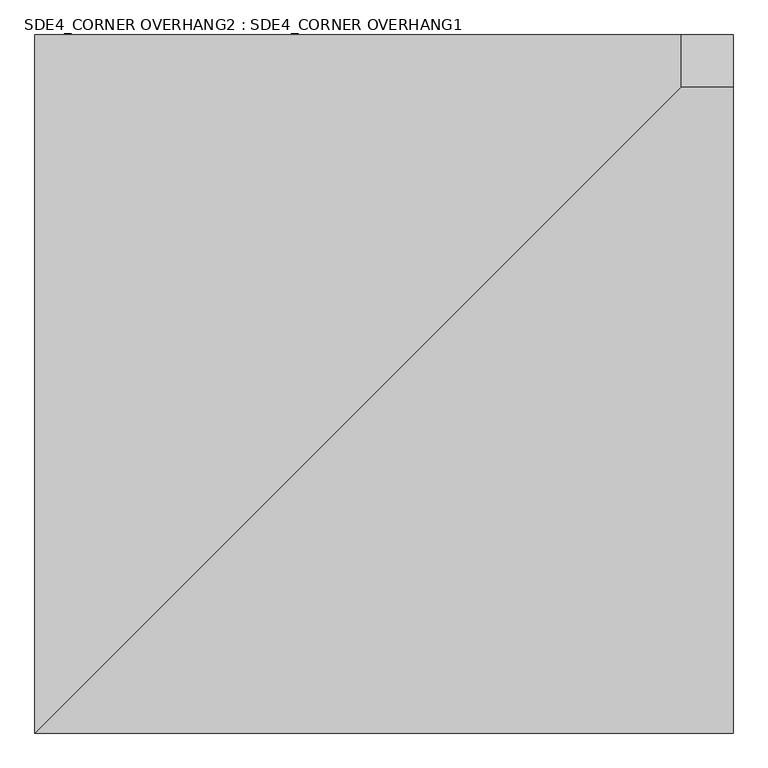
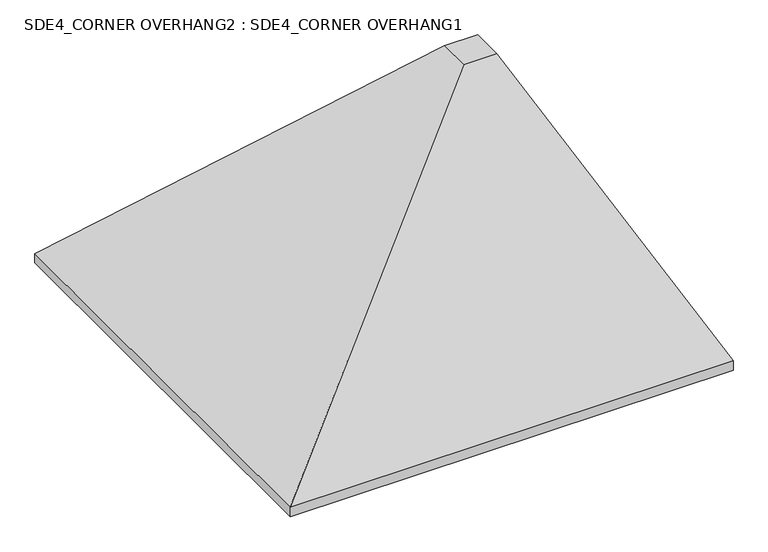
"""IFC4 building model written with IfcOpenShell, lengths in millimetres: proxy geometry, SDE4_CORNER OVERHANG2 : SDE4_CORNER OVERHANG1."""

from ifc_helpers import new_model, si_unit, origin, place, context, project, spatial, faceted_brep, source, transform, mapped, element, save


def sde4_corner_overhang2_sde4_corner_overhang1_35c641b1(model_context):
    return source(origin(), model_context, "Body", "Brep", [
        faceted_brep([(1305.0, -1544.7500001, 142560.0), (1305.0, -1544.7500001, 142520.0), (3105.0, -1544.7500001, 142520.0), (3105.0, -1544.7500001, 142560.0), (2970.0, 255.2499999, 142870.0), (3105.0, 255.2499999, 142870.0), (3105.0, 255.2499999, 142520.0), (1305.0, 255.2499999, 142520.0), (1305.0, 255.2499999, 142560.0), (3105.0, 120.2499999, 142870.0), (2970.0, 120.2499999, 142870.0)], [[[0, 1, 2, 3]], [[4, 5, 6, 7, 8]], [[6, 5, 9, 3, 2]], [[2, 1, 7, 6]], [[1, 0, 8, 7]], [[4, 8, 0, 10]], [[0, 3, 9, 10]], [[5, 4, 10, 9]]]),
    ])


if __name__ == "__main__":
    model = new_model("IFC4")
    model_context = context("Model", 3, world=origin())
    ifc_project = project(units=[si_unit("LENGTHUNIT", "METRE", prefix="MILLI")], contexts=[model_context])
    site = spatial("IfcSite", under=ifc_project)
    building = spatial("IfcBuilding", under=site)
    placement = place(None, origin())
    sde4_corner_overhang2_sde4_corner_overhang1_shape = sde4_corner_overhang2_sde4_corner_overhang1_35c641b1(model_context)
    element("IfcBuildingElementProxy", 1, Name="SDE4_CORNER OVERHANG2 : SDE4_CORNER OVERHANG1", ObjectType="SDE4_CORNER OVERHANG2 : SDE4_CORNER OVERHANG1", at=placement, inside=building, context=model_context, shape_type="MappedRepresentation", body=[
        mapped(sde4_corner_overhang2_sde4_corner_overhang1_shape, transform((0.0, 0.0, 0.0), x_axis=(1.0, 0.0, 0.0), y_axis=(0.0, 1.0, 0.0), z_axis=(0.0, 0.0, 1.0))),
    ])
    save(model, "model.ifc")
